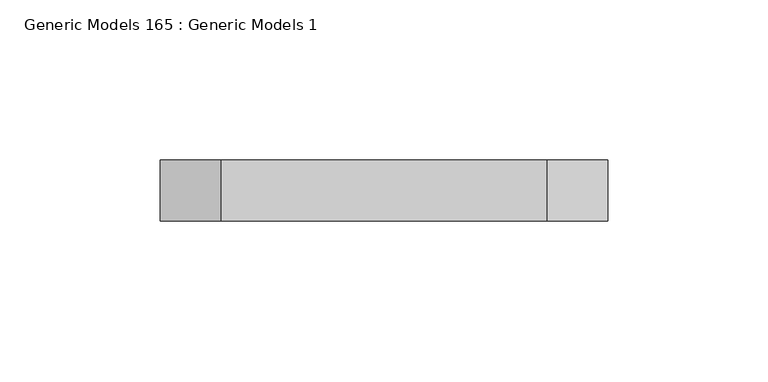
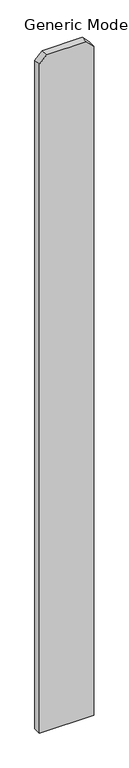
"""IFC4 building model written with IfcOpenShell, lengths in millimetres: proxy geometry, Generic Models 165 : Generic Models 1."""

import ifcopenshell
import ifcopenshell.guid

model = None  # the IFC model being written
_history = None  # IfcOwnerHistory: only IFC2X3 demands one
_inside = {}  # id of a spatial element -> (the spatial element, [elements in it])
_under = {}  # id of a project, library or spatial element -> (it, [spatial elements below it])
_declared = {}  # id of a project -> (the project, [libraries it declares])
_typed = {}  # id of a type object -> (the type object, [elements of that type])
_made_of = {}  # id of a material, layer set ... -> (it, [elements and type objects made of it])


def new_model(schema):
    """Start an empty IFC model of exactly this schema.

    Asked for "IFC4X3", IfcOpenShell would pick the latest addendum, in which some entities
    have other attributes; the version numbers below select the first issue.
    IFC2X3 requires an IfcOwnerHistory on every rooted entity: one is made here for all.
    """
    global model, _history
    if schema == "IFC4X3":
        model = ifcopenshell.file(schema_version=(4, 3, 0, 0))
    else:
        model = ifcopenshell.file(schema=schema)
    _inside.clear()
    _under.clear()
    _declared.clear()
    _typed.clear()
    _made_of.clear()
    _history = None
    if model.schema == "IFC2X3":
        org = make("IfcOrganization", Name="unknown")
        user = make(
            "IfcPersonAndOrganization",
            ThePerson=make("IfcPerson", FamilyName="unknown"),
            TheOrganization=org,
        )
        app = make(
            "IfcApplication",
            ApplicationDeveloper=org,
            Version="unknown",
            ApplicationFullName="unknown",
            ApplicationIdentifier="unknown",
        )
        _history = make(
            "IfcOwnerHistory",
            OwningUser=user,
            OwningApplication=app,
            ChangeAction="ADDED",
            CreationDate=0,
        )
    return model


def make(cls, **values):
    """One entity of the class cls with the attributes given. An attribute that is None is left unset."""
    return model.create_entity(
        cls, **{name: value for name, value in values.items() if value is not None}
    )


def rooted(cls, **values):
    """An entity with a GlobalId (a new one), such as an element, a storey or a relation."""
    return make(cls, GlobalId=ifcopenshell.guid.new(), OwnerHistory=_history, **values)


def si_unit(unit_type, name, prefix=None):
    """IfcSIUnit, for example si_unit("LENGTHUNIT", "METRE", prefix="MILLI")."""
    return make("IfcSIUnit", UnitType=unit_type, Prefix=prefix, Name=name)


def assignment(units):
    """IfcUnitAssignment: the units of a project."""
    return None if units is None else make("IfcUnitAssignment", Units=units)


def point(xyz):
    """IfcCartesianPoint."""
    return None if xyz is None else make("IfcCartesianPoint", Coordinates=xyz)


def direction(xyz):
    """IfcDirection."""
    return None if xyz is None else make("IfcDirection", DirectionRatios=xyz)


def frame(location, z_axis=None, x_axis=None):
    """IfcAxis2Placement3D, a coordinate frame: its origin and axes. An axis left out is left unset."""
    return make(
        "IfcAxis2Placement3D",
        Location=point(location),
        Axis=direction(z_axis),
        RefDirection=direction(x_axis),
    )


def origin():
    """The frame at (0, 0, 0) with its axes left unset."""
    return frame((0.0, 0.0, 0.0))


def place(relative_to, where):
    """IfcLocalPlacement: puts the frame where relative to a parent placement (None: the world)."""
    return make(
        "IfcLocalPlacement", PlacementRelTo=relative_to, RelativePlacement=where
    )


def context(
    kind, dimensions, precision=None, world=None, true_north=None, identifier=None
):
    """IfcGeometricRepresentationContext, for example the 3D "Model" context."""
    return make(
        "IfcGeometricRepresentationContext",
        ContextIdentifier=identifier,
        ContextType=kind,
        CoordinateSpaceDimension=dimensions,
        Precision=precision,
        WorldCoordinateSystem=world,
        TrueNorth=true_north,
    )


def project(units=None, contexts=None):
    """IfcProject with its units and contexts."""
    return rooted(
        "IfcProject",
        Name="project",
        RepresentationContexts=contexts,
        UnitsInContext=assignment(units),
    )


def spatial(cls, under=None, at=None, **own):
    """A site, building, storey or space (cls), placed at a placement, below another one or the project."""
    s = rooted(cls, ObjectPlacement=at, **own)
    if under is not None:
        _under.setdefault(under.id(), (under, []))[1].append(s)
    return s


def polyline(points):
    """IfcPolyline through the points."""
    return make("IfcPolyline", Points=[point(p) for p in points])


def outline(outer, holes=None, kind="AREA"):
    """IfcArbitraryClosedProfileDef: a profile drawn as a closed curve; with holes, ...WithVoids."""
    if holes is None:
        return make("IfcArbitraryClosedProfileDef", ProfileType=kind, OuterCurve=outer)
    return make(
        "IfcArbitraryProfileDefWithVoids",
        ProfileType=kind,
        OuterCurve=outer,
        InnerCurves=holes,
    )


def extrude(swept, where, along, depth):
    """IfcExtrudedAreaSolid: the profile swept, set in the frame where, extruded along a direction by depth."""
    return make(
        "IfcExtrudedAreaSolid",
        SweptArea=swept,
        Position=where,
        ExtrudedDirection=direction(along),
        Depth=depth,
    )


def shape(context_of_items, identifier, shape_type, items):
    """IfcShapeRepresentation: the items that make up one representation, for example the "Body"."""
    return make(
        "IfcShapeRepresentation",
        ContextOfItems=context_of_items,
        RepresentationIdentifier=identifier,
        RepresentationType=shape_type,
        Items=items,
    )


def source(mapping_origin, context_of_items, identifier, shape_type, items):
    """IfcRepresentationMap: a shape defined once, which mapped items show again and again."""
    return make(
        "IfcRepresentationMap",
        MappingOrigin=mapping_origin,
        MappedRepresentation=shape(context_of_items, identifier, shape_type, items),
    )


def transform(
    local_origin,
    x_axis=None,
    y_axis=None,
    z_axis=None,
    scale=None,
    scale2=None,
    scale3=None,
    uniform=True,
):
    """IfcCartesianTransformationOperator3D, or its non-uniform kind. x_axis, y_axis, z_axis: its Axis1, 2, 3."""
    if uniform:
        return make(
            "IfcCartesianTransformationOperator3D",
            Axis1=direction(x_axis),
            Axis2=direction(y_axis),
            LocalOrigin=point(local_origin),
            Scale=scale,
            Axis3=direction(z_axis),
        )
    return make(
        "IfcCartesianTransformationOperator3DnonUniform",
        Axis1=direction(x_axis),
        Axis2=direction(y_axis),
        LocalOrigin=point(local_origin),
        Scale=scale,
        Axis3=direction(z_axis),
        Scale2=scale2,
        Scale3=scale3,
    )


def mapped(mapping_source, mapping_target):
    """IfcMappedItem: shows the shape of a source again, moved by a transform."""
    return make(
        "IfcMappedItem", MappingSource=mapping_source, MappingTarget=mapping_target
    )


def made_of(thing, what):
    """Note that an element or type object is made of a material, layer set ...; save() writes the relation."""
    if what is not None:
        _made_of.setdefault(what.id(), (what, []))[1].append(thing)
    return thing


def element(
    cls,
    number,
    at=None,
    inside=None,
    cuts=None,
    type_object=None,
    material=None,
    context=None,
    identifier="Body",
    shape_type=None,
    held_by="IfcProductDefinitionShape",
    body=None,
    shapes=None,
    **own,
):
    """One element of the class cls, such as IfcWall. Its Tag is "e" and its number.

    at: its placement. inside: the storey or other place that contains it. cuts: it is an
    opening in that element (IfcRelVoidsElement). A single representation is given by context,
    identifier, shape_type and body (its items); several are given by shapes. held_by: the class
    of the entity that holds the representations. save() writes the other relations.
    """
    e = rooted(cls, Tag="e%d" % number, ObjectPlacement=at, **own)
    if body is not None:
        shapes = [shape(context, identifier, shape_type, body)]
    if shapes is not None:
        e.Representation = make(held_by, Representations=shapes)
    if inside is not None:
        _inside.setdefault(inside.id(), (inside, []))[1].append(e)
    if cuts is not None:
        rooted(
            "IfcRelVoidsElement", RelatingBuildingElement=cuts, RelatedOpeningElement=e
        )
    if type_object is not None:
        _typed.setdefault(type_object.id(), (type_object, []))[1].append(e)
    return made_of(e, material)


def aggregate(whole, parts):
    """IfcRelAggregates: a whole, such as a stair, and the parts it consists of."""
    return rooted("IfcRelAggregates", RelatingObject=whole, RelatedObjects=parts)


def save(model, path):
    """Write the relations noted so far, then the file.

    IfcRelAggregates (storeys below a building ...), IfcRelContainedInSpatialStructure (elements
    in a storey), IfcRelDefinesByType, IfcRelAssociatesMaterial and IfcRelDeclares: one each for
    every whole, place, type object, material and project.
    """
    for whole, parts in _under.values():
        aggregate(whole, parts)
    for where, things in _inside.values():
        rooted(
            "IfcRelContainedInSpatialStructure",
            RelatedElements=things,
            RelatingStructure=where,
        )
    for kind, things in _typed.values():
        rooted("IfcRelDefinesByType", RelatedObjects=things, RelatingType=kind)
    for what, things in _made_of.values():
        rooted("IfcRelAssociatesMaterial", RelatedObjects=things, RelatingMaterial=what)
    for by, libraries in _declared.values():
        rooted("IfcRelDeclares", RelatingContext=by, RelatedDefinitions=libraries)
    model.write(path)


def generic_models_165_generic_models_1_5969d6cb(model_context):
    return source(origin(), model_context, "Body", "SweptSolid", [
        extrude(outline(polyline([(76.2, 55141.8125), (1885.95, 55141.8125), (1905.0, 55122.7625), (1905.0, 55021.1625), (1885.95, 55002.1125), (76.2, 55002.1125), (76.2, 55141.8125)])), frame((0.0, 547.6875, 0.0), z_axis=(0.0, 1.0, 0.0), x_axis=(0.0, 0.0, 1.0)), (0.0, 0.0, 1.0), 19.05),
    ])


if __name__ == "__main__":
    model = new_model("IFC4")
    model_context = context("Model", 3, world=origin())
    ifc_project = project(units=[si_unit("LENGTHUNIT", "METRE", prefix="MILLI")], contexts=[model_context])
    site = spatial("IfcSite", under=ifc_project)
    building = spatial("IfcBuilding", under=site)
    placement = place(None, origin())
    generic_models_165_generic_models_1_shape = generic_models_165_generic_models_1_5969d6cb(model_context)
    element("IfcBuildingElementProxy", 1, Name="Generic Models 165 : Generic Models 1", ObjectType="Generic Models 165 : Generic Models 1", at=placement, inside=building, context=model_context, shape_type="MappedRepresentation", body=[
        mapped(generic_models_165_generic_models_1_shape, transform((0.0, 0.0, 0.0), x_axis=(1.0, 0.0, 0.0), y_axis=(0.0, 1.0, 0.0), z_axis=(0.0, 0.0, 1.0))),
    ])
    save(model, "model.ifc")

# Revit data of these elements
# Project information
#   Project Issue Date = "06/12/2018"
#   Project Status = "Project Status"
#   Client Name = "Owner"
#   Project Address = "5253 KING JAMES WAY, FITCHBURG, WI"
#   Project Name = "FORAGE KOMBUCHA"
#   Project Number = "Project Number"
# Element 1 (IfcBuildingElementProxy, "Generic Models 165 : Generic Models 1")
#   Materials on its faces: "VERTICAL 1X6 CEDAR PLANKS W/ CLEAR WOOD SEALER"
# Materials
#   "VERTICAL 1X6 CEDAR PLANKS W/ CLEAR WOOD SEALER": class "Wood", colour RGB 234 198 147, transparency 0, Description = "Pinus Echinata", Cost = 0
